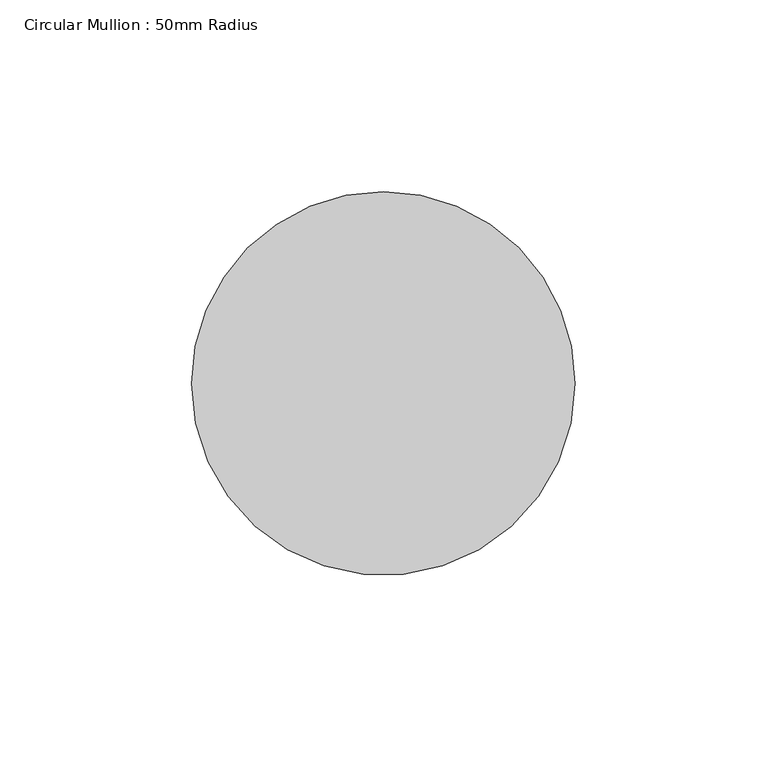
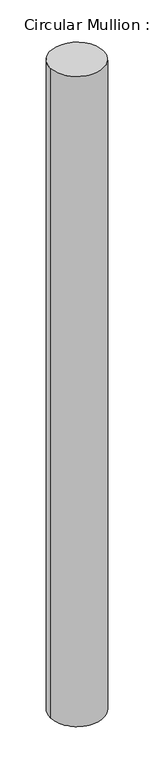
"""IFC4 building model written with IfcOpenShell, lengths in millimetres: member geometry, Circular Mullion : 50mm Radius."""

from ifc_helpers import new_model, si_unit, frame, origin, place, context, project, spatial, ellipse_curve, source, transform, mapped, element, save
from ifc_brep_helpers import plane_surface, cylinder_surface, advanced_brep


def circular_mullion_50mm_radius_8ffe4b28(model_context):
    return source(origin(), model_context, "Body", "AdvancedBrep", [
        advanced_brep(
        [(-100.0, 0.0, 0.6250089), (0.0, 0.0, 0.0), (0.0, 0.0, -1288.8208774), (-100.0, 0.0, -1289.4867576)],
        [
            (0, 1, ellipse_curve(frame((-50.0, 0.0, 0.3125044), z_axis=(-0.006249106887064453, -0.01658611134698799, -0.9998429124485002), x_axis=(-0.35251767622630076, -0.9356372895099403, 0.017724289167716515)), 50.0078556, 50.0)),
            (1, 2),
            (2, 3, ellipse_curve(frame((-50.0, 0.0, -1289.1538175), z_axis=(-0.006657614971868446, -0.017670355976367267, 0.9998217014460903), x_axis=(0.352510197798217, 0.9356174405871328, 0.018882937203862565)), 50.0089165, 50.0)),
            (3, 0),
            (1, 0, ellipse_curve(frame((-50.0, 0.0, 0.3125044), z_axis=(-0.006249106887064453, -0.01658611134698799, -0.9998429124485002), x_axis=(-0.35251767622630076, -0.9356372895099403, 0.017724289167716515)), 50.0078556, 50.0)),
            (3, 2, ellipse_curve(frame((-50.0, 0.0, -1289.1538175), z_axis=(-0.006657614971868446, -0.017670355976367267, 0.9998217014460903), x_axis=(0.352510197798217, 0.9356174405871328, 0.018882937203862565)), 50.0089165, 50.0)),
        ],
        [
            cylinder_surface(frame((-50.0, 0.0, 0.0), z_axis=(0.0, 0.0, 1.0), x_axis=(1.0, 0.0, 0.0)), 50.0),
            plane_surface(frame((-285.2270515, 107.464269, 0.0), z_axis=(0.006249106887064455, 0.016586111346987994, 0.9998429124485004), x_axis=(0.35251767622630087, 0.9356372895099406, -0.01772428916771108))),
            plane_surface(frame((-285.2270515, 107.464269, -1288.8208774), z_axis=(0.006657614971868448, 0.01767035597636727, -0.9998217014460905), x_axis=(0.3525101977982171, 0.9356174405871328, 0.018882937203867023))),
        ],
        [
            (0, [[1, 2, 3, 4]]),
            (0, [[5, -4, 6, -2]]),
            (1, [[-1, -5]]),
            (2, [[-6, -3]]),
        ],
    ),
    ])


if __name__ == "__main__":
    model = new_model("IFC4")
    model_context = context("Model", 3, world=origin())
    ifc_project = project(units=[si_unit("LENGTHUNIT", "METRE", prefix="MILLI")], contexts=[model_context])
    site = spatial("IfcSite", under=ifc_project)
    building = spatial("IfcBuilding", under=site)
    placement = place(None, origin())
    circular_mullion_50mm_radius_shape = circular_mullion_50mm_radius_8ffe4b28(model_context)
    element("IfcMember", 1, ObjectType="Circular Mullion : 50mm Radius", at=placement, inside=building, context=model_context, shape_type="MappedRepresentation", body=[
        mapped(circular_mullion_50mm_radius_shape, transform((0.0, 0.0, 0.0), x_axis=(1.0, 0.0, 0.0), y_axis=(0.0, 1.0, 0.0), z_axis=(0.0, 0.0, 1.0))),
    ])
    save(model, "model.ifc")

# Revit data of these elements
# Type "Circular Mullion : 50mm Radius"
#   built-in parameter 1007350 = 0.164042 (stored number, unit not read)
# Element 1 (IfcMember, "Circular Mullion : 50mm Radius")
#   Materials on its faces: "Aluminium"
# Materials
#   "Aluminium": class "Metal", colour RGB 247 247 247, transparency 0, Description = "Aluminium 6061", Cost = 0
